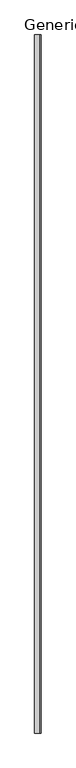
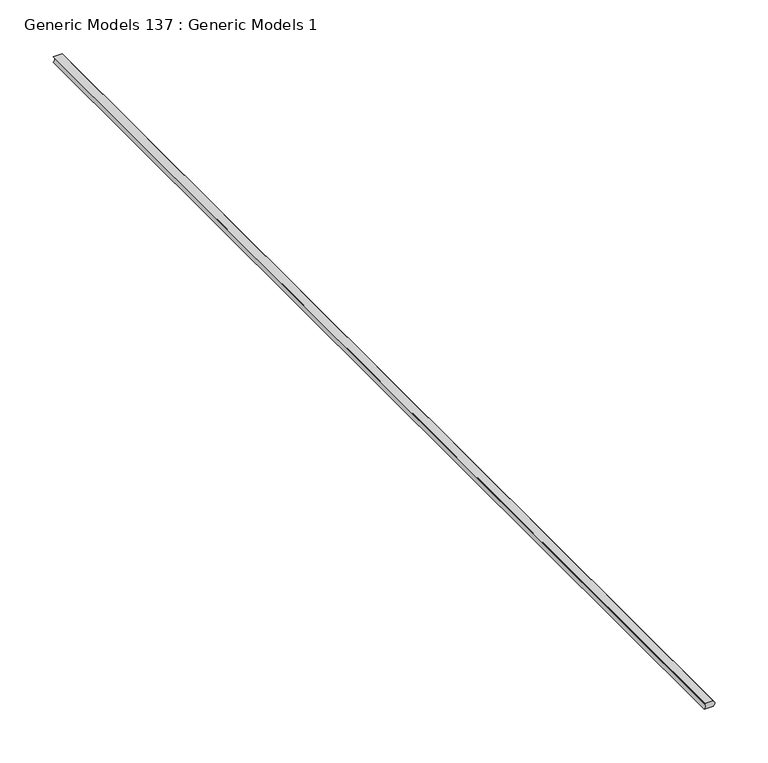
"""IFC4 building model written with IfcOpenShell, lengths in millimetres: proxy geometry, Generic Models 137 : Generic Models 1."""

import ifcopenshell
import ifcopenshell.guid

model = None  # the IFC model being written
_history = None  # IfcOwnerHistory: only IFC2X3 demands one
_inside = {}  # id of a spatial element -> (the spatial element, [elements in it])
_under = {}  # id of a project, library or spatial element -> (it, [spatial elements below it])
_declared = {}  # id of a project -> (the project, [libraries it declares])
_typed = {}  # id of a type object -> (the type object, [elements of that type])
_made_of = {}  # id of a material, layer set ... -> (it, [elements and type objects made of it])


def new_model(schema):
    """Start an empty IFC model of exactly this schema.

    Asked for "IFC4X3", IfcOpenShell would pick the latest addendum, in which some entities
    have other attributes; the version numbers below select the first issue.
    IFC2X3 requires an IfcOwnerHistory on every rooted entity: one is made here for all.
    """
    global model, _history
    if schema == "IFC4X3":
        model = ifcopenshell.file(schema_version=(4, 3, 0, 0))
    else:
        model = ifcopenshell.file(schema=schema)
    _inside.clear()
    _under.clear()
    _declared.clear()
    _typed.clear()
    _made_of.clear()
    _history = None
    if model.schema == "IFC2X3":
        org = make("IfcOrganization", Name="unknown")
        user = make(
            "IfcPersonAndOrganization",
            ThePerson=make("IfcPerson", FamilyName="unknown"),
            TheOrganization=org,
        )
        app = make(
            "IfcApplication",
            ApplicationDeveloper=org,
            Version="unknown",
            ApplicationFullName="unknown",
            ApplicationIdentifier="unknown",
        )
        _history = make(
            "IfcOwnerHistory",
            OwningUser=user,
            OwningApplication=app,
            ChangeAction="ADDED",
            CreationDate=0,
        )
    return model


def make(cls, **values):
    """One entity of the class cls with the attributes given. An attribute that is None is left unset."""
    return model.create_entity(
        cls, **{name: value for name, value in values.items() if value is not None}
    )


def rooted(cls, **values):
    """An entity with a GlobalId (a new one), such as an element, a storey or a relation."""
    return make(cls, GlobalId=ifcopenshell.guid.new(), OwnerHistory=_history, **values)


def si_unit(unit_type, name, prefix=None):
    """IfcSIUnit, for example si_unit("LENGTHUNIT", "METRE", prefix="MILLI")."""
    return make("IfcSIUnit", UnitType=unit_type, Prefix=prefix, Name=name)


def assignment(units):
    """IfcUnitAssignment: the units of a project."""
    return None if units is None else make("IfcUnitAssignment", Units=units)


def point(xyz):
    """IfcCartesianPoint."""
    return None if xyz is None else make("IfcCartesianPoint", Coordinates=xyz)


def direction(xyz):
    """IfcDirection."""
    return None if xyz is None else make("IfcDirection", DirectionRatios=xyz)


def frame(location, z_axis=None, x_axis=None):
    """IfcAxis2Placement3D, a coordinate frame: its origin and axes. An axis left out is left unset."""
    return make(
        "IfcAxis2Placement3D",
        Location=point(location),
        Axis=direction(z_axis),
        RefDirection=direction(x_axis),
    )


def frame_2d(location, x_axis=None):
    """IfcAxis2Placement2D, a coordinate frame in the plane: its origin and x axis."""
    return make(
        "IfcAxis2Placement2D", Location=point(location), RefDirection=direction(x_axis)
    )


def origin():
    """The frame at (0, 0, 0) with its axes left unset."""
    return frame((0.0, 0.0, 0.0))


def place(relative_to, where):
    """IfcLocalPlacement: puts the frame where relative to a parent placement (None: the world)."""
    return make(
        "IfcLocalPlacement", PlacementRelTo=relative_to, RelativePlacement=where
    )


def context(
    kind, dimensions, precision=None, world=None, true_north=None, identifier=None
):
    """IfcGeometricRepresentationContext, for example the 3D "Model" context."""
    return make(
        "IfcGeometricRepresentationContext",
        ContextIdentifier=identifier,
        ContextType=kind,
        CoordinateSpaceDimension=dimensions,
        Precision=precision,
        WorldCoordinateSystem=world,
        TrueNorth=true_north,
    )


def project(units=None, contexts=None):
    """IfcProject with its units and contexts."""
    return rooted(
        "IfcProject",
        Name="project",
        RepresentationContexts=contexts,
        UnitsInContext=assignment(units),
    )


def spatial(cls, under=None, at=None, **own):
    """A site, building, storey or space (cls), placed at a placement, below another one or the project."""
    s = rooted(cls, ObjectPlacement=at, **own)
    if under is not None:
        _under.setdefault(under.id(), (under, []))[1].append(s)
    return s


def polyline(points):
    """IfcPolyline through the points."""
    return make("IfcPolyline", Points=[point(p) for p in points])


def circle_curve(where, radius):
    """IfcCircle in the frame where."""
    return make("IfcCircle", Position=where, Radius=radius)


def trimmed(basis, trim1, trim2, sense, master):
    """IfcTrimmedCurve: the piece of a basis curve between two trims."""
    return make(
        "IfcTrimmedCurve",
        BasisCurve=basis,
        Trim1=trim1,
        Trim2=trim2,
        SenseAgreement=sense,
        MasterRepresentation=master,
    )


def segment(curve, same_sense, transition):
    """IfcCompositeCurveSegment."""
    return make(
        "IfcCompositeCurveSegment",
        Transition=transition,
        SameSense=same_sense,
        ParentCurve=curve,
    )


def composite_curve(segments, self_intersect=None):
    """IfcCompositeCurve: segments joined end to end."""
    return make("IfcCompositeCurve", Segments=segments, SelfIntersect=self_intersect)


def outline(outer, holes=None, kind="AREA"):
    """IfcArbitraryClosedProfileDef: a profile drawn as a closed curve; with holes, ...WithVoids."""
    if holes is None:
        return make("IfcArbitraryClosedProfileDef", ProfileType=kind, OuterCurve=outer)
    return make(
        "IfcArbitraryProfileDefWithVoids",
        ProfileType=kind,
        OuterCurve=outer,
        InnerCurves=holes,
    )


def extrude(swept, where, along, depth):
    """IfcExtrudedAreaSolid: the profile swept, set in the frame where, extruded along a direction by depth."""
    return make(
        "IfcExtrudedAreaSolid",
        SweptArea=swept,
        Position=where,
        ExtrudedDirection=direction(along),
        Depth=depth,
    )


def shape(context_of_items, identifier, shape_type, items):
    """IfcShapeRepresentation: the items that make up one representation, for example the "Body"."""
    return make(
        "IfcShapeRepresentation",
        ContextOfItems=context_of_items,
        RepresentationIdentifier=identifier,
        RepresentationType=shape_type,
        Items=items,
    )


def source(mapping_origin, context_of_items, identifier, shape_type, items):
    """IfcRepresentationMap: a shape defined once, which mapped items show again and again."""
    return make(
        "IfcRepresentationMap",
        MappingOrigin=mapping_origin,
        MappedRepresentation=shape(context_of_items, identifier, shape_type, items),
    )


def transform(
    local_origin,
    x_axis=None,
    y_axis=None,
    z_axis=None,
    scale=None,
    scale2=None,
    scale3=None,
    uniform=True,
):
    """IfcCartesianTransformationOperator3D, or its non-uniform kind. x_axis, y_axis, z_axis: its Axis1, 2, 3."""
    if uniform:
        return make(
            "IfcCartesianTransformationOperator3D",
            Axis1=direction(x_axis),
            Axis2=direction(y_axis),
            LocalOrigin=point(local_origin),
            Scale=scale,
            Axis3=direction(z_axis),
        )
    return make(
        "IfcCartesianTransformationOperator3DnonUniform",
        Axis1=direction(x_axis),
        Axis2=direction(y_axis),
        LocalOrigin=point(local_origin),
        Scale=scale,
        Axis3=direction(z_axis),
        Scale2=scale2,
        Scale3=scale3,
    )


def mapped(mapping_source, mapping_target):
    """IfcMappedItem: shows the shape of a source again, moved by a transform."""
    return make(
        "IfcMappedItem", MappingSource=mapping_source, MappingTarget=mapping_target
    )


def made_of(thing, what):
    """Note that an element or type object is made of a material, layer set ...; save() writes the relation."""
    if what is not None:
        _made_of.setdefault(what.id(), (what, []))[1].append(thing)
    return thing


def element(
    cls,
    number,
    at=None,
    inside=None,
    cuts=None,
    type_object=None,
    material=None,
    context=None,
    identifier="Body",
    shape_type=None,
    held_by="IfcProductDefinitionShape",
    body=None,
    shapes=None,
    **own,
):
    """One element of the class cls, such as IfcWall. Its Tag is "e" and its number.

    at: its placement. inside: the storey or other place that contains it. cuts: it is an
    opening in that element (IfcRelVoidsElement). A single representation is given by context,
    identifier, shape_type and body (its items); several are given by shapes. held_by: the class
    of the entity that holds the representations. save() writes the other relations.
    """
    e = rooted(cls, Tag="e%d" % number, ObjectPlacement=at, **own)
    if body is not None:
        shapes = [shape(context, identifier, shape_type, body)]
    if shapes is not None:
        e.Representation = make(held_by, Representations=shapes)
    if inside is not None:
        _inside.setdefault(inside.id(), (inside, []))[1].append(e)
    if cuts is not None:
        rooted(
            "IfcRelVoidsElement", RelatingBuildingElement=cuts, RelatedOpeningElement=e
        )
    if type_object is not None:
        _typed.setdefault(type_object.id(), (type_object, []))[1].append(e)
    return made_of(e, material)


def aggregate(whole, parts):
    """IfcRelAggregates: a whole, such as a stair, and the parts it consists of."""
    return rooted("IfcRelAggregates", RelatingObject=whole, RelatedObjects=parts)


def save(model, path):
    """Write the relations noted so far, then the file.

    IfcRelAggregates (storeys below a building ...), IfcRelContainedInSpatialStructure (elements
    in a storey), IfcRelDefinesByType, IfcRelAssociatesMaterial and IfcRelDeclares: one each for
    every whole, place, type object, material and project.
    """
    for whole, parts in _under.values():
        aggregate(whole, parts)
    for where, things in _inside.values():
        rooted(
            "IfcRelContainedInSpatialStructure",
            RelatedElements=things,
            RelatingStructure=where,
        )
    for kind, things in _typed.values():
        rooted("IfcRelDefinesByType", RelatedObjects=things, RelatingType=kind)
    for what, things in _made_of.values():
        rooted("IfcRelAssociatesMaterial", RelatedObjects=things, RelatingMaterial=what)
    for by, libraries in _declared.values():
        rooted("IfcRelDeclares", RelatingContext=by, RelatedDefinitions=libraries)
    model.write(path)


def generic_models_137_generic_models_1_9cb7df0c(model_context):
    return source(origin(), model_context, "Body", "SweptSolid", [
        extrude(outline(composite_curve([segment(polyline([(-225.976067, 48050.3548058), (-225.976067, 48059.8798058)]), True, "CONTINUOUS"), segment(trimmed(circle_curve(frame_2d((-222.801067, 48056.9650653)), 4.3100275), [point((-225.976067, 48059.8798058))], [point((-219.626067, 48059.8798058))], False, "CARTESIAN"), True, "CONTINUOUS"), segment(polyline([(-219.626067, 48059.8798058), (-219.626067, 48050.3548058)]), True, "CONTINUOUS"), segment(trimmed(circle_curve(frame_2d((-222.801067, 48047.4400653)), 4.3100275), [point((-219.626067, 48050.3548058))], [point((-225.976067, 48050.3548058))], True, "CARTESIAN"), True, "CONTINUOUS")], self_intersect=False)), frame((0.0, 0.0, 0.0), z_axis=(0.0, 1.0, 0.0), x_axis=(0.0, 0.0, 1.0)), (0.0, 0.0, 1.0), 1219.2),
    ])


if __name__ == "__main__":
    model = new_model("IFC4")
    model_context = context("Model", 3, world=origin())
    ifc_project = project(units=[si_unit("LENGTHUNIT", "METRE", prefix="MILLI")], contexts=[model_context])
    site = spatial("IfcSite", under=ifc_project)
    building = spatial("IfcBuilding", under=site)
    placement = place(None, origin())
    generic_models_137_generic_models_1_shape = generic_models_137_generic_models_1_9cb7df0c(model_context)
    element("IfcBuildingElementProxy", 1, Name="Generic Models 137 : Generic Models 1", ObjectType="Generic Models 137 : Generic Models 1", at=placement, inside=building, context=model_context, shape_type="MappedRepresentation", body=[
        mapped(generic_models_137_generic_models_1_shape, transform((0.0, 0.0, 0.0), x_axis=(1.0, 0.0, 0.0), y_axis=(0.0, 1.0, 0.0), z_axis=(0.0, 0.0, 1.0))),
    ])
    save(model, "model.ifc")

# Revit data of these elements
# Element 1 (IfcBuildingElementProxy, "Generic Models 137 : Generic Models 1")
#   Materials on its faces: "SEALANT (W/ BACKER ROD IF NECESSARY)"
# Materials
#   "SEALANT (W/ BACKER ROD IF NECESSARY)": class "Unassigned", colour RGB 120 120 120, transparency 0, Cost = 0
